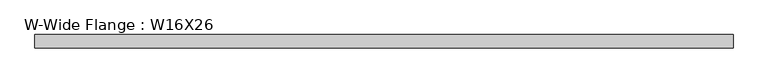
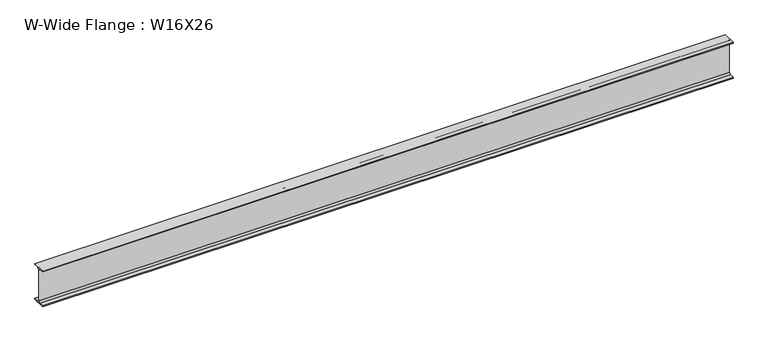
"""IFC4 building model written with IfcOpenShell, lengths in millimetres: beam geometry, W-Wide Flange : W16X26."""

from ifc_helpers import new_model, si_unit, point, frame, frame_2d, origin, place, context, project, spatial, polyline, circle_curve, trimmed, segment, composite_curve, outline, extrude, source, transform, mapped, element, save


def w_wide_flange_w16x26_1ab7282a(model_context):
    return source(origin(), model_context, "Body", "SweptSolid", [
        extrude(outline(composite_curve([segment(polyline([(69.85, -190.627), (69.85, -199.39), (-69.85, -199.39), (-69.85, -190.627), (-21.3995, -190.627)]), True, "CONTINUOUS"), segment(trimmed(circle_curve(frame_2d((-21.3995, -172.4025)), 18.2245), [point((-21.3995, -190.627))], [point((-3.175, -172.4025))], True, "CARTESIAN"), True, "CONTINUOUS"), segment(polyline([(-3.175, -172.4025), (-3.175, 172.4025)]), True, "CONTINUOUS"), segment(trimmed(circle_curve(frame_2d((-21.3995, 172.4025)), 18.2245), [point((-3.175, 172.4025))], [point((-21.3995, 190.627))], True, "CARTESIAN"), True, "CONTINUOUS"), segment(polyline([(-21.3995, 190.627), (-69.85, 190.627), (-69.85, 199.39), (69.85, 199.39), (69.85, 190.627), (21.3995, 190.627)]), True, "CONTINUOUS"), segment(trimmed(circle_curve(frame_2d((21.3995, 172.4025)), 18.2245), [point((21.3995, 190.627))], [point((3.175, 172.4025))], True, "CARTESIAN"), True, "CONTINUOUS"), segment(polyline([(3.175, 172.4025), (3.175, -172.4025)]), True, "CONTINUOUS"), segment(trimmed(circle_curve(frame_2d((21.3995, -172.4025)), 18.2245), [point((3.175, -172.4025))], [point((21.3995, -190.627))], True, "CARTESIAN"), True, "CONTINUOUS"), segment(polyline([(21.3995, -190.627), (69.85, -190.627)]), True, "CONTINUOUS")], self_intersect=False)), frame((-3657.6015875, 0.0, 0.0), z_axis=(1.0, 0.0, 0.0), x_axis=(0.0, 1.0, 0.0)), (0.0, 0.0, 1.0), 7315.203175),
    ])


if __name__ == "__main__":
    model = new_model("IFC4")
    model_context = context("Model", 3, world=origin())
    ifc_project = project(units=[si_unit("LENGTHUNIT", "METRE", prefix="MILLI")], contexts=[model_context])
    site = spatial("IfcSite", under=ifc_project)
    building = spatial("IfcBuilding", under=site)
    placement = place(None, origin())
    w_wide_flange_w16x26_shape = w_wide_flange_w16x26_1ab7282a(model_context)
    element("IfcBeam", 1, ObjectType="W-Wide Flange : W16X26", at=placement, inside=building, context=model_context, shape_type="MappedRepresentation", body=[
        mapped(w_wide_flange_w16x26_shape, transform((0.0, 0.0, 0.0), x_axis=(1.0, 0.0, 0.0), y_axis=(0.0, 1.0, 0.0), z_axis=(0.0, 0.0, 1.0))),
    ])
    save(model, "model.ifc")

# Revit data of these elements
# Type "W-Wide Flange : W16X26"
#   Assembly Code = "B10"
#   W = 26
#   Length [instance default] = 5' - 0"
#   bf = 0' - 5 1/2"
#   d = 1' - 3.7"
#   k = 0' - 1 1/16"
#   k2 = 0' - 0.7175"
#   tf = 0' - 0.345"
#   tw = 0' - 0 1/4"
#   A = 0.0533333 SF
#   Structural Material [instance default] = Steel ASTM A992
# Element 1 (IfcBeam, "W-Wide Flange : W16X26")
#   Structural Material = none
# Materials
#   "Steel ASTM A992": class "Metal", colour RGB 189 187 185, transparency 0, Description = "Structural steel 50ksi", Cost = 0
